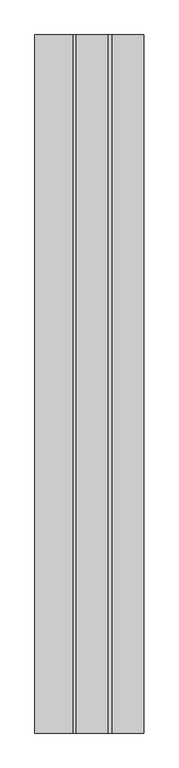
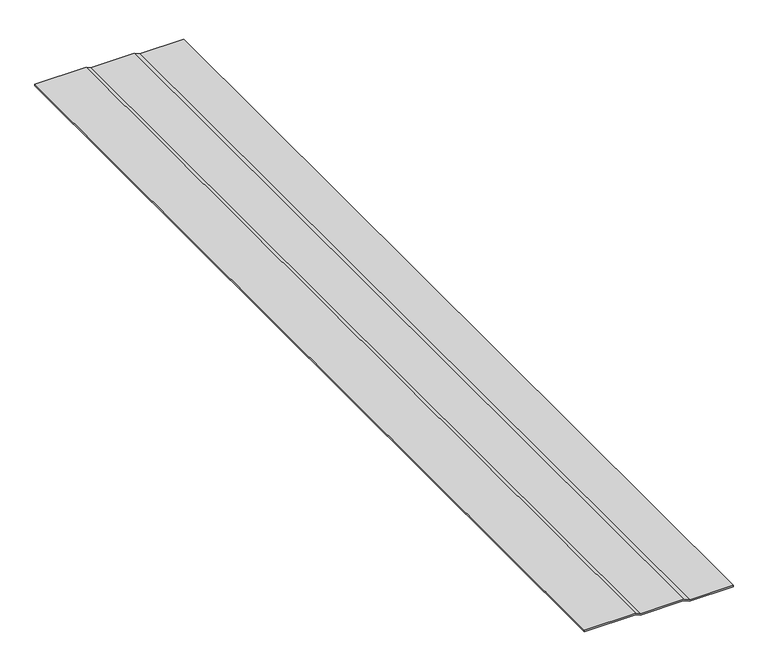
"""IFC4 building model written with IfcOpenShell, lengths in millimetres: proxy geometry, BITUMEN CAP SHEET003 14655 : BITUMEN CAP SHEET003 14655."""

import ifcopenshell
import ifcopenshell.guid

model = None  # the IFC model being written
_history = None  # IfcOwnerHistory: only IFC2X3 demands one
_inside = {}  # id of a spatial element -> (the spatial element, [elements in it])
_under = {}  # id of a project, library or spatial element -> (it, [spatial elements below it])
_declared = {}  # id of a project -> (the project, [libraries it declares])
_typed = {}  # id of a type object -> (the type object, [elements of that type])
_made_of = {}  # id of a material, layer set ... -> (it, [elements and type objects made of it])


def new_model(schema):
    """Start an empty IFC model of exactly this schema.

    Asked for "IFC4X3", IfcOpenShell would pick the latest addendum, in which some entities
    have other attributes; the version numbers below select the first issue.
    IFC2X3 requires an IfcOwnerHistory on every rooted entity: one is made here for all.
    """
    global model, _history
    if schema == "IFC4X3":
        model = ifcopenshell.file(schema_version=(4, 3, 0, 0))
    else:
        model = ifcopenshell.file(schema=schema)
    _inside.clear()
    _under.clear()
    _declared.clear()
    _typed.clear()
    _made_of.clear()
    _history = None
    if model.schema == "IFC2X3":
        org = make("IfcOrganization", Name="unknown")
        user = make(
            "IfcPersonAndOrganization",
            ThePerson=make("IfcPerson", FamilyName="unknown"),
            TheOrganization=org,
        )
        app = make(
            "IfcApplication",
            ApplicationDeveloper=org,
            Version="unknown",
            ApplicationFullName="unknown",
            ApplicationIdentifier="unknown",
        )
        _history = make(
            "IfcOwnerHistory",
            OwningUser=user,
            OwningApplication=app,
            ChangeAction="ADDED",
            CreationDate=0,
        )
    return model


def make(cls, **values):
    """One entity of the class cls with the attributes given. An attribute that is None is left unset."""
    return model.create_entity(
        cls, **{name: value for name, value in values.items() if value is not None}
    )


def rooted(cls, **values):
    """An entity with a GlobalId (a new one), such as an element, a storey or a relation."""
    return make(cls, GlobalId=ifcopenshell.guid.new(), OwnerHistory=_history, **values)


def si_unit(unit_type, name, prefix=None):
    """IfcSIUnit, for example si_unit("LENGTHUNIT", "METRE", prefix="MILLI")."""
    return make("IfcSIUnit", UnitType=unit_type, Prefix=prefix, Name=name)


def assignment(units):
    """IfcUnitAssignment: the units of a project."""
    return None if units is None else make("IfcUnitAssignment", Units=units)


def point(xyz):
    """IfcCartesianPoint."""
    return None if xyz is None else make("IfcCartesianPoint", Coordinates=xyz)


def direction(xyz):
    """IfcDirection."""
    return None if xyz is None else make("IfcDirection", DirectionRatios=xyz)


def frame(location, z_axis=None, x_axis=None):
    """IfcAxis2Placement3D, a coordinate frame: its origin and axes. An axis left out is left unset."""
    return make(
        "IfcAxis2Placement3D",
        Location=point(location),
        Axis=direction(z_axis),
        RefDirection=direction(x_axis),
    )


def origin():
    """The frame at (0, 0, 0) with its axes left unset."""
    return frame((0.0, 0.0, 0.0))


def place(relative_to, where):
    """IfcLocalPlacement: puts the frame where relative to a parent placement (None: the world)."""
    return make(
        "IfcLocalPlacement", PlacementRelTo=relative_to, RelativePlacement=where
    )


def context(
    kind, dimensions, precision=None, world=None, true_north=None, identifier=None
):
    """IfcGeometricRepresentationContext, for example the 3D "Model" context."""
    return make(
        "IfcGeometricRepresentationContext",
        ContextIdentifier=identifier,
        ContextType=kind,
        CoordinateSpaceDimension=dimensions,
        Precision=precision,
        WorldCoordinateSystem=world,
        TrueNorth=true_north,
    )


def project(units=None, contexts=None):
    """IfcProject with its units and contexts."""
    return rooted(
        "IfcProject",
        Name="project",
        RepresentationContexts=contexts,
        UnitsInContext=assignment(units),
    )


def spatial(cls, under=None, at=None, **own):
    """A site, building, storey or space (cls), placed at a placement, below another one or the project."""
    s = rooted(cls, ObjectPlacement=at, **own)
    if under is not None:
        _under.setdefault(under.id(), (under, []))[1].append(s)
    return s


def polyline(points):
    """IfcPolyline through the points."""
    return make("IfcPolyline", Points=[point(p) for p in points])


def outline(outer, holes=None, kind="AREA"):
    """IfcArbitraryClosedProfileDef: a profile drawn as a closed curve; with holes, ...WithVoids."""
    if holes is None:
        return make("IfcArbitraryClosedProfileDef", ProfileType=kind, OuterCurve=outer)
    return make(
        "IfcArbitraryProfileDefWithVoids",
        ProfileType=kind,
        OuterCurve=outer,
        InnerCurves=holes,
    )


def extrude(swept, where, along, depth):
    """IfcExtrudedAreaSolid: the profile swept, set in the frame where, extruded along a direction by depth."""
    return make(
        "IfcExtrudedAreaSolid",
        SweptArea=swept,
        Position=where,
        ExtrudedDirection=direction(along),
        Depth=depth,
    )


def shape(context_of_items, identifier, shape_type, items):
    """IfcShapeRepresentation: the items that make up one representation, for example the "Body"."""
    return make(
        "IfcShapeRepresentation",
        ContextOfItems=context_of_items,
        RepresentationIdentifier=identifier,
        RepresentationType=shape_type,
        Items=items,
    )


def source(mapping_origin, context_of_items, identifier, shape_type, items):
    """IfcRepresentationMap: a shape defined once, which mapped items show again and again."""
    return make(
        "IfcRepresentationMap",
        MappingOrigin=mapping_origin,
        MappedRepresentation=shape(context_of_items, identifier, shape_type, items),
    )


def transform(
    local_origin,
    x_axis=None,
    y_axis=None,
    z_axis=None,
    scale=None,
    scale2=None,
    scale3=None,
    uniform=True,
):
    """IfcCartesianTransformationOperator3D, or its non-uniform kind. x_axis, y_axis, z_axis: its Axis1, 2, 3."""
    if uniform:
        return make(
            "IfcCartesianTransformationOperator3D",
            Axis1=direction(x_axis),
            Axis2=direction(y_axis),
            LocalOrigin=point(local_origin),
            Scale=scale,
            Axis3=direction(z_axis),
        )
    return make(
        "IfcCartesianTransformationOperator3DnonUniform",
        Axis1=direction(x_axis),
        Axis2=direction(y_axis),
        LocalOrigin=point(local_origin),
        Scale=scale,
        Axis3=direction(z_axis),
        Scale2=scale2,
        Scale3=scale3,
    )


def mapped(mapping_source, mapping_target):
    """IfcMappedItem: shows the shape of a source again, moved by a transform."""
    return make(
        "IfcMappedItem", MappingSource=mapping_source, MappingTarget=mapping_target
    )


def made_of(thing, what):
    """Note that an element or type object is made of a material, layer set ...; save() writes the relation."""
    if what is not None:
        _made_of.setdefault(what.id(), (what, []))[1].append(thing)
    return thing


def element(
    cls,
    number,
    at=None,
    inside=None,
    cuts=None,
    type_object=None,
    material=None,
    context=None,
    identifier="Body",
    shape_type=None,
    held_by="IfcProductDefinitionShape",
    body=None,
    shapes=None,
    **own,
):
    """One element of the class cls, such as IfcWall. Its Tag is "e" and its number.

    at: its placement. inside: the storey or other place that contains it. cuts: it is an
    opening in that element (IfcRelVoidsElement). A single representation is given by context,
    identifier, shape_type and body (its items); several are given by shapes. held_by: the class
    of the entity that holds the representations. save() writes the other relations.
    """
    e = rooted(cls, Tag="e%d" % number, ObjectPlacement=at, **own)
    if body is not None:
        shapes = [shape(context, identifier, shape_type, body)]
    if shapes is not None:
        e.Representation = make(held_by, Representations=shapes)
    if inside is not None:
        _inside.setdefault(inside.id(), (inside, []))[1].append(e)
    if cuts is not None:
        rooted(
            "IfcRelVoidsElement", RelatingBuildingElement=cuts, RelatedOpeningElement=e
        )
    if type_object is not None:
        _typed.setdefault(type_object.id(), (type_object, []))[1].append(e)
    return made_of(e, material)


def aggregate(whole, parts):
    """IfcRelAggregates: a whole, such as a stair, and the parts it consists of."""
    return rooted("IfcRelAggregates", RelatingObject=whole, RelatedObjects=parts)


def save(model, path):
    """Write the relations noted so far, then the file.

    IfcRelAggregates (storeys below a building ...), IfcRelContainedInSpatialStructure (elements
    in a storey), IfcRelDefinesByType, IfcRelAssociatesMaterial and IfcRelDeclares: one each for
    every whole, place, type object, material and project.
    """
    for whole, parts in _under.values():
        aggregate(whole, parts)
    for where, things in _inside.values():
        rooted(
            "IfcRelContainedInSpatialStructure",
            RelatedElements=things,
            RelatingStructure=where,
        )
    for kind, things in _typed.values():
        rooted("IfcRelDefinesByType", RelatedObjects=things, RelatingType=kind)
    for what, things in _made_of.values():
        rooted("IfcRelAssociatesMaterial", RelatedObjects=things, RelatingMaterial=what)
    for by, libraries in _declared.values():
        rooted("IfcRelDeclares", RelatingContext=by, RelatedDefinitions=libraries)
    model.write(path)


def generic_models_03d49bda(model_context):
    return source(origin(), model_context, "Body", "SweptSolid", [
        extrude(outline(polyline([(40259.2002678, -2469.2761954), (40262.3752678, -2469.2761954), (40262.3752678, -2560.795457), (40267.6612773, -2573.2602756), (40267.6612773, -2663.9440313), (40271.9940719, -2673.6609328), (40271.9940719, -2781.5474293), (40268.8188423, -2781.5474293), (40268.8188423, -2674.3362183), (40264.4862773, -2664.6198318), (40264.4862773, -2573.9056756), (40259.2002678, -2561.440857), (40259.2002678, -2469.2761954)])), frame((0.0, 999.75, 0.0), z_axis=(0.0, 1.0, 0.0), x_axis=(0.0, 0.0, 1.0)), (0.0, 0.0, 1.0), 2000.25),
    ])


if __name__ == "__main__":
    model = new_model("IFC4")
    model_context = context("Model", 3, world=origin())
    ifc_project = project(units=[si_unit("LENGTHUNIT", "METRE", prefix="MILLI")], contexts=[model_context])
    site = spatial("IfcSite", under=ifc_project)
    building = spatial("IfcBuilding", under=site)
    placement = place(None, origin())
    generic_models_shape = generic_models_03d49bda(model_context)
    element("IfcBuildingElementProxy", 1, Name="BITUMEN CAP SHEET003 14655 : BITUMEN CAP SHEET003 14655", ObjectType="BITUMEN CAP SHEET003 14655 : BITUMEN CAP SHEET003 14655", at=placement, inside=building, context=model_context, shape_type="MappedRepresentation", body=[
        mapped(generic_models_shape, transform((0.0, 0.0, 0.0), x_axis=(1.0, 0.0, 0.0), y_axis=(0.0, 1.0, 0.0), z_axis=(0.0, 0.0, 1.0))),
    ])
    save(model, "model.ifc")

# Revit data of these elements
# Project information
#   Issued Date 1 = "0/00/2018 - City of Newport Beach"
#   IfcSite GUID = "3elgjS7H4HwQsE093rt3ko"
#   IfcBuilding GUID = "3eliBW7H4HwQsE093rt3ko"
#   IfcProject GUID = "3580753c_1e44_4e66_87a"
#   NameOverride = "Default Site"
#   Project Issue Date = "Issue Date"
#   Project Status = "Project Status"
#   Client Name = "xxx"
#   Project Address = "xxx"
#   Project Name = "STAUDENMEIER RESIDENCE"
# Type "BITUMEN CAP SHEET003 14655 : BITUMEN CAP SHEET003 14655"
#   NameOverride = "BITUMEN CAP SHEET003"
# Element 1 (IfcBuildingElementProxy, "BITUMEN CAP SHEET003 14655 : BITUMEN CAP SHEET003 14655")
#   Materials on its faces: "MODIFIED BITUMEN GRANULE SURFACED CAP SHEET"
# Materials
#   "MODIFIED BITUMEN GRANULE SURFACED CAP SHEET": class "Unassigned", colour RGB 85 85 127, transparency 0
